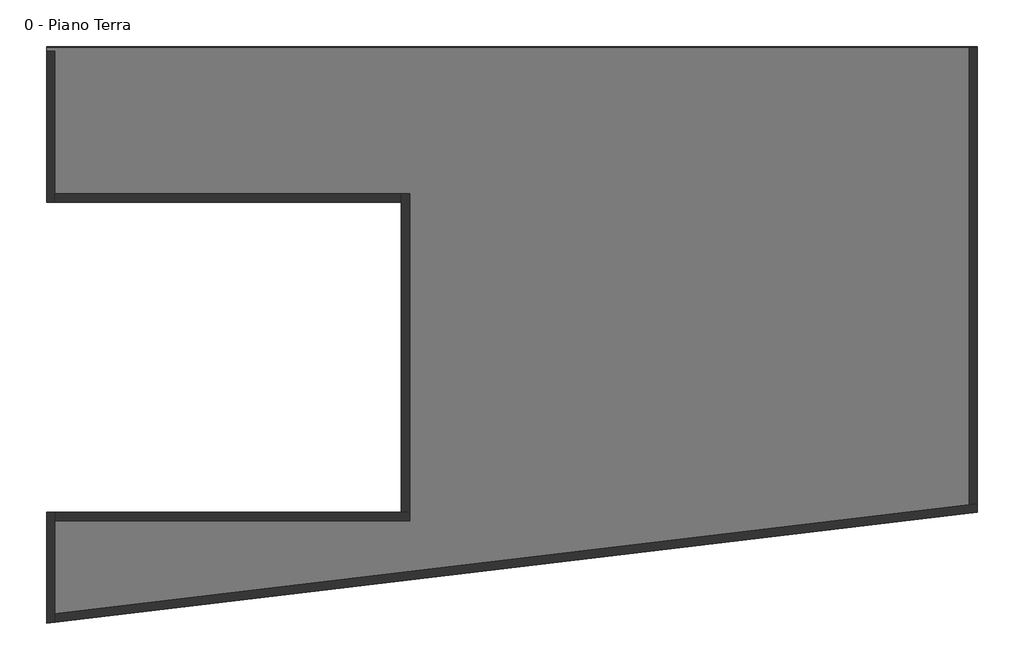
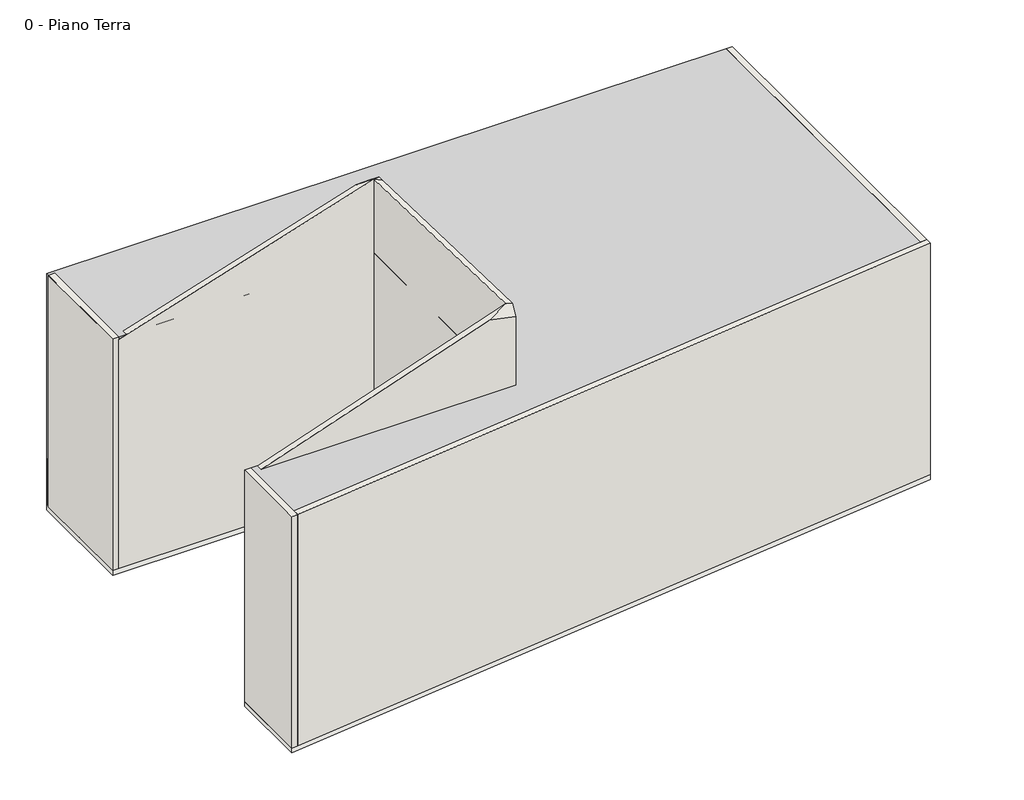
# One storey: 7 walls, 5 plates, 1 proxy, 1 slab.
"""IFC4 building model written with IfcOpenShell, lengths in millimetres."""

import ifcopenshell
import ifcopenshell.guid

model = None  # the IFC model being written
_history = None  # IfcOwnerHistory: only IFC2X3 demands one
_inside = {}  # id of a spatial element -> (the spatial element, [elements in it])
_under = {}  # id of a project, library or spatial element -> (it, [spatial elements below it])
_declared = {}  # id of a project -> (the project, [libraries it declares])
_typed = {}  # id of a type object -> (the type object, [elements of that type])
_made_of = {}  # id of a material, layer set ... -> (it, [elements and type objects made of it])


def new_model(schema):
    """Start an empty IFC model of exactly this schema.

    Asked for "IFC4X3", IfcOpenShell would pick the latest addendum, in which some entities
    have other attributes; the version numbers below select the first issue.
    IFC2X3 requires an IfcOwnerHistory on every rooted entity: one is made here for all.
    """
    global model, _history
    if schema == "IFC4X3":
        model = ifcopenshell.file(schema_version=(4, 3, 0, 0))
    else:
        model = ifcopenshell.file(schema=schema)
    _inside.clear()
    _under.clear()
    _declared.clear()
    _typed.clear()
    _made_of.clear()
    _history = None
    if model.schema == "IFC2X3":
        org = make("IfcOrganization", Name="unknown")
        user = make(
            "IfcPersonAndOrganization",
            ThePerson=make("IfcPerson", FamilyName="unknown"),
            TheOrganization=org,
        )
        app = make(
            "IfcApplication",
            ApplicationDeveloper=org,
            Version="unknown",
            ApplicationFullName="unknown",
            ApplicationIdentifier="unknown",
        )
        _history = make(
            "IfcOwnerHistory",
            OwningUser=user,
            OwningApplication=app,
            ChangeAction="ADDED",
            CreationDate=0,
        )
    return model


def make(cls, **values):
    """One entity of the class cls with the attributes given. An attribute that is None is left unset."""
    return model.create_entity(
        cls, **{name: value for name, value in values.items() if value is not None}
    )


def rooted(cls, **values):
    """An entity with a GlobalId (a new one), such as an element, a storey or a relation."""
    return make(cls, GlobalId=ifcopenshell.guid.new(), OwnerHistory=_history, **values)


def si_unit(unit_type, name, prefix=None):
    """IfcSIUnit, for example si_unit("LENGTHUNIT", "METRE", prefix="MILLI")."""
    return make("IfcSIUnit", UnitType=unit_type, Prefix=prefix, Name=name)


def assignment(units):
    """IfcUnitAssignment: the units of a project."""
    return None if units is None else make("IfcUnitAssignment", Units=units)


def point(xyz):
    """IfcCartesianPoint."""
    return None if xyz is None else make("IfcCartesianPoint", Coordinates=xyz)


def direction(xyz):
    """IfcDirection."""
    return None if xyz is None else make("IfcDirection", DirectionRatios=xyz)


def frame(location, z_axis=None, x_axis=None):
    """IfcAxis2Placement3D, a coordinate frame: its origin and axes. An axis left out is left unset."""
    return make(
        "IfcAxis2Placement3D",
        Location=point(location),
        Axis=direction(z_axis),
        RefDirection=direction(x_axis),
    )


def origin():
    """The frame at (0, 0, 0) with its axes left unset."""
    return frame((0.0, 0.0, 0.0))


def origin_with_axes():
    """The frame at (0, 0, 0) with the z axis (0, 0, 1) and the x axis (1, 0, 0) written out."""
    return frame((0.0, 0.0, 0.0), z_axis=(0.0, 0.0, 1.0), x_axis=(1.0, 0.0, 0.0))


def place(relative_to, where):
    """IfcLocalPlacement: puts the frame where relative to a parent placement (None: the world)."""
    return make(
        "IfcLocalPlacement", PlacementRelTo=relative_to, RelativePlacement=where
    )


def context(
    kind, dimensions, precision=None, world=None, true_north=None, identifier=None
):
    """IfcGeometricRepresentationContext, for example the 3D "Model" context."""
    return make(
        "IfcGeometricRepresentationContext",
        ContextIdentifier=identifier,
        ContextType=kind,
        CoordinateSpaceDimension=dimensions,
        Precision=precision,
        WorldCoordinateSystem=world,
        TrueNorth=true_north,
    )


def project(units=None, contexts=None):
    """IfcProject with its units and contexts."""
    return rooted(
        "IfcProject",
        Name="project",
        RepresentationContexts=contexts,
        UnitsInContext=assignment(units),
    )


def spatial(cls, under=None, at=None, **own):
    """A site, building, storey or space (cls), placed at a placement, below another one or the project."""
    s = rooted(cls, ObjectPlacement=at, **own)
    if under is not None:
        _under.setdefault(under.id(), (under, []))[1].append(s)
    return s


def polyline(points):
    """IfcPolyline through the points."""
    return make("IfcPolyline", Points=[point(p) for p in points])


def outline(outer, holes=None, kind="AREA"):
    """IfcArbitraryClosedProfileDef: a profile drawn as a closed curve; with holes, ...WithVoids."""
    if holes is None:
        return make("IfcArbitraryClosedProfileDef", ProfileType=kind, OuterCurve=outer)
    return make(
        "IfcArbitraryProfileDefWithVoids",
        ProfileType=kind,
        OuterCurve=outer,
        InnerCurves=holes,
    )


def extrude(swept, where, along, depth):
    """IfcExtrudedAreaSolid: the profile swept, set in the frame where, extruded along a direction by depth."""
    return make(
        "IfcExtrudedAreaSolid",
        SweptArea=swept,
        Position=where,
        ExtrudedDirection=direction(along),
        Depth=depth,
    )


def faces_of(points, faces, orient=None, outer=None):
    """IfcFace entities. A face is a list of loops; a loop is a list of indices into points, from 0.

    orient and outer hold one flag for each loop. By default every Orientation is true, the
    first loop of a face is its IfcFaceOuterBound and the others are IfcFaceBound.
    """
    made = []
    for i, loops in enumerate(faces):
        bounds = []
        for j, loop in enumerate(loops):
            is_outer = j == 0 if outer is None else outer[i][j]
            bounds.append(
                make(
                    "IfcFaceOuterBound" if is_outer else "IfcFaceBound",
                    Bound=make("IfcPolyLoop", Polygon=[points[k] for k in loop]),
                    Orientation=True if orient is None else orient[i][j],
                )
            )
        made.append(make("IfcFace", Bounds=bounds))
    return made


def faceted_brep(points, faces, orient=None, outer=None, voids=None):
    """IfcFacetedBrep: a solid bounded by flat faces; with voids (closed shells), ...WithVoids."""
    shared = [point(p) for p in points]
    hull = make("IfcClosedShell", CfsFaces=faces_of(shared, faces, orient, outer))
    if voids is None:
        return make("IfcFacetedBrep", Outer=hull)
    return make(
        "IfcFacetedBrepWithVoids",
        Outer=hull,
        Voids=[
            make(cls, CfsFaces=faces_of(shared, fs, o, b)) for cls, fs, o, b in voids
        ],
    )


def shape(context_of_items, identifier, shape_type, items):
    """IfcShapeRepresentation: the items that make up one representation, for example the "Body"."""
    return make(
        "IfcShapeRepresentation",
        ContextOfItems=context_of_items,
        RepresentationIdentifier=identifier,
        RepresentationType=shape_type,
        Items=items,
    )


def source(mapping_origin, context_of_items, identifier, shape_type, items):
    """IfcRepresentationMap: a shape defined once, which mapped items show again and again."""
    return make(
        "IfcRepresentationMap",
        MappingOrigin=mapping_origin,
        MappedRepresentation=shape(context_of_items, identifier, shape_type, items),
    )


def transform(
    local_origin,
    x_axis=None,
    y_axis=None,
    z_axis=None,
    scale=None,
    scale2=None,
    scale3=None,
    uniform=True,
):
    """IfcCartesianTransformationOperator3D, or its non-uniform kind. x_axis, y_axis, z_axis: its Axis1, 2, 3."""
    if uniform:
        return make(
            "IfcCartesianTransformationOperator3D",
            Axis1=direction(x_axis),
            Axis2=direction(y_axis),
            LocalOrigin=point(local_origin),
            Scale=scale,
            Axis3=direction(z_axis),
        )
    return make(
        "IfcCartesianTransformationOperator3DnonUniform",
        Axis1=direction(x_axis),
        Axis2=direction(y_axis),
        LocalOrigin=point(local_origin),
        Scale=scale,
        Axis3=direction(z_axis),
        Scale2=scale2,
        Scale3=scale3,
    )


def mapped(mapping_source, mapping_target):
    """IfcMappedItem: shows the shape of a source again, moved by a transform."""
    return make(
        "IfcMappedItem", MappingSource=mapping_source, MappingTarget=mapping_target
    )


def made_of(thing, what):
    """Note that an element or type object is made of a material, layer set ...; save() writes the relation."""
    if what is not None:
        _made_of.setdefault(what.id(), (what, []))[1].append(thing)
    return thing


def element(
    cls,
    number,
    at=None,
    inside=None,
    cuts=None,
    type_object=None,
    material=None,
    context=None,
    identifier="Body",
    shape_type=None,
    held_by="IfcProductDefinitionShape",
    body=None,
    shapes=None,
    **own,
):
    """One element of the class cls, such as IfcWall. Its Tag is "e" and its number.

    at: its placement. inside: the storey or other place that contains it. cuts: it is an
    opening in that element (IfcRelVoidsElement). A single representation is given by context,
    identifier, shape_type and body (its items); several are given by shapes. held_by: the class
    of the entity that holds the representations. save() writes the other relations.
    """
    e = rooted(cls, Tag="e%d" % number, ObjectPlacement=at, **own)
    if body is not None:
        shapes = [shape(context, identifier, shape_type, body)]
    if shapes is not None:
        e.Representation = make(held_by, Representations=shapes)
    if inside is not None:
        _inside.setdefault(inside.id(), (inside, []))[1].append(e)
    if cuts is not None:
        rooted(
            "IfcRelVoidsElement", RelatingBuildingElement=cuts, RelatedOpeningElement=e
        )
    if type_object is not None:
        _typed.setdefault(type_object.id(), (type_object, []))[1].append(e)
    return made_of(e, material)


def aggregate(whole, parts):
    """IfcRelAggregates: a whole, such as a stair, and the parts it consists of."""
    return rooted("IfcRelAggregates", RelatingObject=whole, RelatedObjects=parts)


def save(model, path):
    """Write the relations noted so far, then the file.

    IfcRelAggregates (storeys below a building ...), IfcRelContainedInSpatialStructure (elements
    in a storey), IfcRelDefinesByType, IfcRelAssociatesMaterial and IfcRelDeclares: one each for
    every whole, place, type object, material and project.
    """
    for whole, parts in _under.values():
        aggregate(whole, parts)
    for where, things in _inside.values():
        rooted(
            "IfcRelContainedInSpatialStructure",
            RelatedElements=things,
            RelatingStructure=where,
        )
    for kind, things in _typed.values():
        rooted("IfcRelDefinesByType", RelatedObjects=things, RelatingType=kind)
    for what, things in _made_of.values():
        rooted("IfcRelAssociatesMaterial", RelatedObjects=things, RelatingMaterial=what)
    for by, libraries in _declared.values():
        rooted("IfcRelDeclares", RelatingContext=by, RelatedDefinitions=libraries)
    model.write(path)


def pannello_sistema_vetrato_29ff3466(model_context):
    return source(origin(), model_context, "Body", "SweptSolid", [
        extrude(outline(polyline([(4200.0000001, -15.0), (-4200.0000001, -15.0), (-4200.0000001, 15.0), (4200.0000001, 15.0), (4200.0000001, -15.0)])), origin_with_axes(), (0.0, 0.0, 1.0), 3000.0),
    ])


model = new_model("IFC4")

# Units and contexts
model_context = context("Model", 3, world=origin())
ifc_project = project(units=[si_unit("LENGTHUNIT", "METRE", prefix="MILLI")], contexts=[model_context])

# Site, building, storey
site = spatial("IfcSite", under=ifc_project)
building = spatial("IfcBuilding", under=site)
storey = spatial("IfcBuildingStorey", under=building, Name="0 - Piano Terra", Elevation=0.0)

# Proxy
placement = place(None, origin())
element("IfcBuildingElementProxy", 1, Name="Famiglia1 : Famiglia1", ObjectType="Famiglia1 : Famiglia1", at=placement, inside=storey, context=model_context, shape_type="SweptSolid", body=[
    extrude(outline(polyline([(-25134.9893486, -7802.5545265), (-9134.9893486, -7802.5545265), (-9134.9893486, 6197.4454735), (-25134.9893486, 6197.4454735), (-25134.9893486, 13197.4454735), (16865.0106514, 13197.4454735), (16865.0106514, -7802.5545265), (-25134.9893486, -12802.5545265), (-25134.9893486, -7802.5545265)])), origin_with_axes(), (0.0, 0.0, 1.0), 15000.0),
])

# Plates
pannello_sistema_vetrato_shape = pannello_sistema_vetrato_29ff3466(model_context)
element("IfcPlate", 2, ObjectType="Pannello sistema : Vetrato", at=placement, inside=storey, context=model_context, shape_type="MappedRepresentation", body=[
    mapped(pannello_sistema_vetrato_shape, transform((-20934.9893485, 13197.4454735, 0.0), x_axis=(1.0, 0.0, 0.0), y_axis=(0.0, 1.0, 0.0), z_axis=(0.0, 0.0, 1.0))),
])
element("IfcPlate", 3, ObjectType="Pannello sistema : Vetrato", at=placement, inside=storey, context=model_context, shape_type="MappedRepresentation", body=[
    mapped(pannello_sistema_vetrato_shape, transform((-12534.9893485, 13197.4454735, 0.0), x_axis=(1.0, 0.0, 0.0), y_axis=(0.0, 1.0, 0.0), z_axis=(0.0, 0.0, 1.0))),
])
element("IfcPlate", 4, ObjectType="Pannello sistema : Vetrato", at=placement, inside=storey, context=model_context, shape_type="MappedRepresentation", body=[
    mapped(pannello_sistema_vetrato_shape, transform((-4134.9893486, 13197.4454735, 0.0), x_axis=(1.0, 0.0, 0.0), y_axis=(0.0, 1.0, 0.0), z_axis=(0.0, 0.0, 1.0))),
])
element("IfcPlate", 5, ObjectType="Pannello sistema : Vetrato", at=placement, inside=storey, context=model_context, shape_type="MappedRepresentation", body=[
    mapped(pannello_sistema_vetrato_shape, transform((4265.0106513, 13197.4454735, 0.0), x_axis=(1.0, 0.0, 0.0), y_axis=(0.0, 1.0, 0.0), z_axis=(0.0, 0.0, 1.0))),
])
element("IfcPlate", 6, ObjectType="Pannello sistema : Vetrato", at=placement, inside=storey, context=model_context, shape_type="MappedRepresentation", body=[
    mapped(pannello_sistema_vetrato_shape, transform((12665.0106513, 13197.4454735, 0.0), x_axis=(1.0, 0.0, 0.0), y_axis=(0.0, 1.0, 0.0), z_axis=(0.0, 0.0, 1.0))),
])

# Slab
element("IfcSlab", 7, ObjectType="Latero Cementizio - 30 cm", at=placement, inside=storey, context=model_context, shape_type="SweptSolid", body=[
    extrude(outline(polyline([(-25134.9893486, -7802.5545265), (-9134.9893486, -7802.5545265), (-9134.9893486, 6197.4454735), (-25134.9893486, 6197.4454735), (-25134.9893486, 13197.4454735), (16865.0106514, 13197.4454735), (16865.0106514, -7802.5545265), (-25134.9893486, -12802.5545265), (-25134.9893486, -7802.5545265)])), frame((0.0, 0.0, -300.0), z_axis=(0.0, 0.0, 1.0), x_axis=(1.0, 0.0, 0.0)), (0.0, 0.0, 1.0), 300.0),
])

# Walls
element("IfcWall", 8, ObjectType="Tamponamento Esterno - 38 cm", at=placement, inside=storey, context=model_context, shape_type="Brep", body=[
    faceted_brep([(-25134.9893486, 13007.4454735, 0.0), (-25134.9893486, 6197.4454735, 0.0), (-25134.9893486, 6197.4454735, 15000.0), (-25134.9893486, 13007.4454735, 15000.0), (-24754.9893486, 13007.4454735, 0.0), (-24754.9893486, 13007.4454735, 15000.0), (-24754.9893486, 6197.4454735, 15000.0), (-24754.9893486, 6197.4454735, 14849.4372915), (-24754.9893486, 6197.4454735, 0.0), (-24754.9893486, 6577.4454735, 0.0)], [[[0, 1, 2, 3]], [[4, 5, 6, 7, 8, 9]], [[1, 0, 4, 9, 8]], [[3, 2, 6, 5]], [[0, 3, 5, 4]], [[2, 1, 8, 7, 6]]]),
])
element("IfcWall", 9, ObjectType="Tamponamento Esterno - 38 cm", at=placement, inside=storey, context=model_context, shape_type="Brep", body=[
    faceted_brep([(-25134.9893486, -7802.5545265, 0.0), (-25134.9893486, -12802.5545265, 0.0), (-25134.9893486, -12802.5545265, 15000.0), (-25134.9893486, -7802.5545265, 15000.0), (-24754.9893486, -7802.5545265, 0.0), (-24754.9893486, -7802.5545265, 14859.5679543), (-24754.9893486, -7802.5545265, 15000.0), (-24754.9893486, -12374.6331611, 15000.0), (-24754.9893486, -12757.3164313, 15000.0), (-24754.9893486, -12757.3164313, 0.0), (-24754.9893486, -12374.6331611, 0.0), (-24754.9893486, -8182.5545265, 0.0)], [[[0, 1, 2, 3]], [[4, 5, 6, 7, 8, 9, 10, 11]], [[1, 0, 4, 11, 10, 9]], [[3, 2, 8, 7, 6]], [[0, 3, 6, 5, 4]], [[2, 1, 9, 8]]]),
])
element("IfcWall", 10, ObjectType="Tamponamento Esterno - 38 cm", at=placement, inside=storey, context=model_context, shape_type="Brep", body=[
    faceted_brep([(-8754.9893486, -7802.5545265, 0.0), (-9134.9893486, -7802.5545265, 0.0), (-24754.9893486, -7802.5545265, 0.0), (-24754.9893486, -7802.5545265, 14859.5679543), (-9134.9893486, -7802.5545265, 20185.4928107), (-8754.9893486, -7802.5545265, 20105.758685), (-8754.9893486, -8182.5545265, 0.0), (-8754.9893486, -8182.5545265, 19435.9920292), (-10350.9893486, -8182.5545265, 19770.8753571), (-24754.9893486, -8182.5545265, 14859.5679543), (-24754.9893486, -8182.5545265, 0.0)], [[[0, 1, 2, 3, 4, 5]], [[6, 7, 8, 9, 10]], [[2, 1, 0, 6, 10]], [[3, 2, 10, 9]], [[0, 5, 7, 6]], [[5, 4, 8, 7]], [[4, 3, 9, 8]]]),
])
element("IfcWall", 11, ObjectType="Tamponamento Esterno - 38 cm", at=placement, inside=storey, context=model_context, shape_type="Brep", body=[
    faceted_brep([(-24754.9893486, -12757.3164313, 0.0), (16865.0106514, -7802.5545265, 0.0), (16865.0106514, -7802.5545265, 15000.0), (-24754.9893486, -12757.3164313, 15000.0), (-24754.9893486, -12374.6331611, 0.0), (-24754.9893486, -12374.6331611, 15000.0), (16485.0106514, -7465.1093516, 15000.0), (16865.0106514, -7419.8712564, 15000.0), (16865.0106514, -7419.8712564, 0.0), (16485.0106514, -7465.1093516, 0.0)], [[[0, 1, 2, 3]], [[4, 5, 6, 7, 8, 9]], [[1, 0, 4, 9, 8]], [[3, 2, 7, 6, 5]], [[0, 3, 5, 4]], [[2, 1, 8, 7]]]),
])
element("IfcWall", 12, ObjectType="Tamponamento Esterno - 38 cm", at=placement, inside=storey, context=model_context, shape_type="SweptSolid", body=[
    extrude(outline(polyline([(16865.0106514, 13212.4454735), (16865.0106514, -7419.8712564), (16485.0106514, -7465.1093516), (16485.0106514, 13212.4454735), (16865.0106514, 13212.4454735)])), origin_with_axes(), (0.0, 0.0, 1.0), 15000.0),
])
element("IfcWall", 13, ObjectType="Tamponamento Esterno - 38 cm", at=placement, inside=storey, context=model_context, shape_type="Brep", body=[
    faceted_brep([(-9134.9893486, 6577.4454735, 0.0), (-9134.9893486, 6197.4454735, 0.0), (-9134.9893486, -7802.5545265, 0.0), (-9134.9893486, -7802.5545265, 20185.4928107), (-9134.9893486, 6197.4454735, 19758.9385911), (-9134.9893486, 6577.4454735, 19485.9390676), (-8754.9893486, 6577.4454735, 0.0), (-8754.9893486, 6577.4454735, 19485.9390676), (-8754.9893486, 6299.7531658, 19685.4387194), (-8754.9893486, 5992.8300888, 19685.4387194), (-8754.9893486, -7802.5545265, 20105.758685), (-8754.9893486, -7802.5545265, 0.0)], [[[0, 1, 2, 3, 4, 5]], [[6, 7, 8, 9, 10, 11]], [[2, 1, 0, 6, 11]], [[3, 2, 11, 10]], [[0, 5, 7, 6]], [[5, 4, 8, 7]], [[4, 3, 10, 9]], [[9, 8, 4]]]),
])
element("IfcWall", 14, ObjectType="Tamponamento Esterno - 38 cm", at=placement, inside=storey, context=model_context, shape_type="Brep", body=[
    faceted_brep([(-24754.9893486, 6197.4454735, 0.0), (-9134.9893486, 6197.4454735, 0.0), (-9134.9893486, 6197.4454735, 19758.9385911), (-24754.9893486, 6197.4454735, 14849.4372915), (-24754.9893486, 6577.4454735, 0.0), (-24754.9893486, 6577.4454735, 14849.4372915), (-10003.5607772, 6577.4454735, 19485.9390676), (-9134.9893486, 6577.4454735, 19485.9390676), (-9134.9893486, 6577.4454735, 0.0)], [[[0, 1, 2, 3]], [[4, 5, 6, 7, 8]], [[1, 0, 4, 8]], [[0, 3, 5, 4]], [[2, 1, 8, 7]], [[3, 2, 6, 5]], [[2, 7, 6]]]),
])

save(model, "model.ifc")

# Revit data of these elements
# Project information
#   Data di consegna del progetto = "Data"
#   Stato del progetto = "Stato"
#   Nome del cliente = "Proprietario"
#   Nome del progetto = "Nome"
#   Numero del progetto = "0001"
# Type "Famiglia1 : Famiglia1"
#   Default Elevation = 1.2192 m
# Type "Pannello sistema : Vetrato"
#   Construction Type Id = "GSP4R"
#   Analytic Construction = "Vetrata singola Pilkington 1/8 in"
#   Visual Light Transmittance = 0.9
#   Solar Heat Gain Coefficient = 0.86
#   Heat Transfer Coefficient (U) = 6.7069 W/(m²·K)
# Type "Latero Cementizio - 30 cm"
#   Keynote = "S/3"
#   Function = 0
#   Layers, outside or top first: 0.02 m "Ceramica bianca" (function 4); 0.065 m "Sabbia e Calcestruzzo" (function 2); 0.04 m "Calcestruzzo" (function 1); 0.16 m "Laterizio (2)" (function 1); 0.015 m "Intonaco - Bianco" (function 5)
# Type "Tamponamento Esterno - 38 cm"
#   Keynote = "Mb/6"
#   Layers, outside or top first: 0.015 m "Intonaco - Beige" (function 4); 0.06 m "Laterizio (5)" (function 2); 0.04 m "Isolamento" (function 3); 0.25 m "Laterizio (4)" (function 1); 0.015 m "Intonaco - Bianco" (function 5)
# Element 1 (IfcBuildingElementProxy, "Famiglia1 : Famiglia1")
#   Phase Created = Stato di Progetto
#   Materials on its faces: "Forma di default"
# Elements 2, 3, 4, 5, 6 (IfcPlate, "Pannello sistema : Vetrato")
#   Phase Created = Stato di Progetto
#   Materials on its faces: "Default - Vetro"
# Element 7 (IfcSlab, "Latero Cementizio - 30 cm")
#   built-in parameter 1001955 = 1.5708 (stored number, unit not read)
#   Height Offset From Level = 0.00 m
#   Phase Created = Stato di Progetto
#   Materials on its faces: "Intonaco - Bianco", "Ceramica bianca"
# Elements 8, 11, 12, 14 (IfcWall, "Tamponamento Esterno - 38 cm")
#   Top Offset = 0.00 m
#   Base Offset = 0.00 m
#   Unconnected Height = 15.00 m
#   wall height = 15.00 m
#   Phase Created = Stato di Progetto
#   Base Constraint = 0 - Piano Terra
#   Materials on its faces: "Default - Calcestruzzo", "Intonaco - Beige", "Intonaco - Bianco"
# Element 9 (IfcWall, "Tamponamento Esterno - 38 cm")
#   Top Offset = 0.00 m
#   Base Offset = 0.00 m
#   Unconnected Height = 15.00 m
#   wall height = 15.00 m
#   Phase Created = Stato di Progetto
#   Base Constraint = 0 - Piano Terra
#   Materials on its faces: "Intonaco - Beige", "Default - Calcestruzzo", "Intonaco - Bianco"
# Elements 10, 13 (IfcWall, "Tamponamento Esterno - 38 cm")
#   Top Offset = 0.00 m
#   Base Offset = 0.00 m
#   Unconnected Height = 15.00 m
#   wall height = 15.00 m
#   Phase Created = Stato di Progetto
#   Base Constraint = 0 - Piano Terra
#   Materials on its faces: "Default - Calcestruzzo", "Intonaco - Bianco", "Intonaco - Beige"
# Materials
#   "Ceramica bianca": class "Ceramica", colour RGB 210 210 210, transparency 0, Description = "Finitura interna - Piastrelle di ceramica incollate", Cost = 0
#   "Sabbia e Calcestruzzo": class "Calcestruzzo", colour RGB 127 127 127, transparency 0, Description = "Magrone - Sabbia e cemento", Cost = 0
#   "Calcestruzzo": class "Calcestruzzo", colour RGB 192 192 192, transparency 0, Description = "Calcestruzzo - Cemento Portland", Cost = 0
#   "Laterizio (2)": class "Mattone", colour RGB 255 128 64, transparency 0, Description = "Pignatta h 16 cm", Cost = 0
#   "Intonaco - Bianco": class "Intonaco", colour RGB 249 249 249, transparency 0, Description = "Verniciatura", Cost = 0
#   "Intonaco - Beige": class "Intonaco", colour RGB 227 215 171, transparency 0, Description = "Verniciatura", Cost = 0
#   "Laterizio (5)": class "Mattone", colour RGB 255 128 64, transparency 0, Description = "Facciata continua 6x25x50 cm", Cost = 0
#   "Isolamento": class "Varie", colour RGB 127 127 127, transparency 0, Description = "Pannello in sughero", Cost = 0
#   "Laterizio (4)": class "Mattone", colour RGB 255 128 64, transparency 0, Description = "Bimattone - 12x12x25 cm", Cost = 0
#   "Forma di default": class "Generico", colour RGB 185 189 196, transparency 0.5, Cost = 0
#   "Default - Vetro": class "Vetro", colour RGB 208 208 208, transparency 0.7, Cost = 0
#   "Default - Calcestruzzo": class "Calcestruzzo", colour RGB 192 192 192, transparency 0, Description = "Calcestruzzo", Cost = 0
